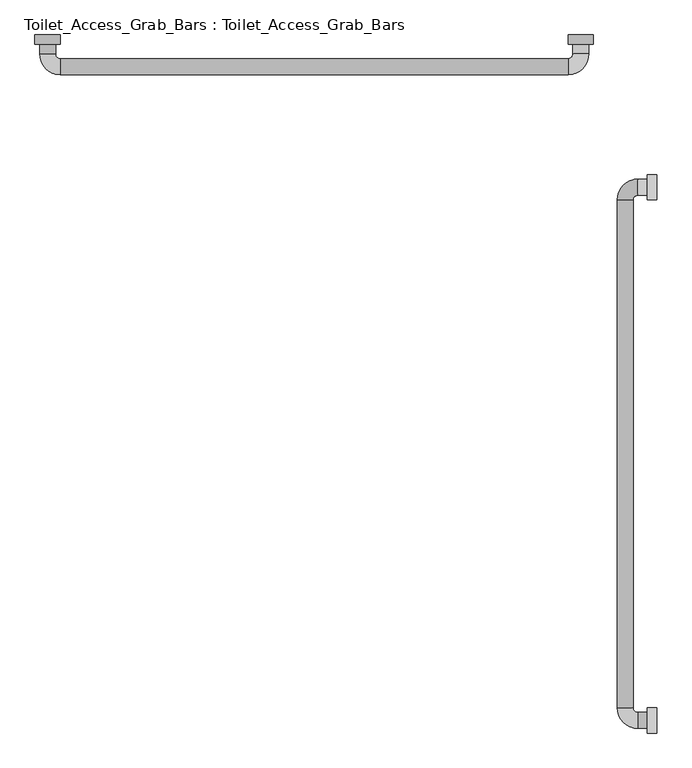
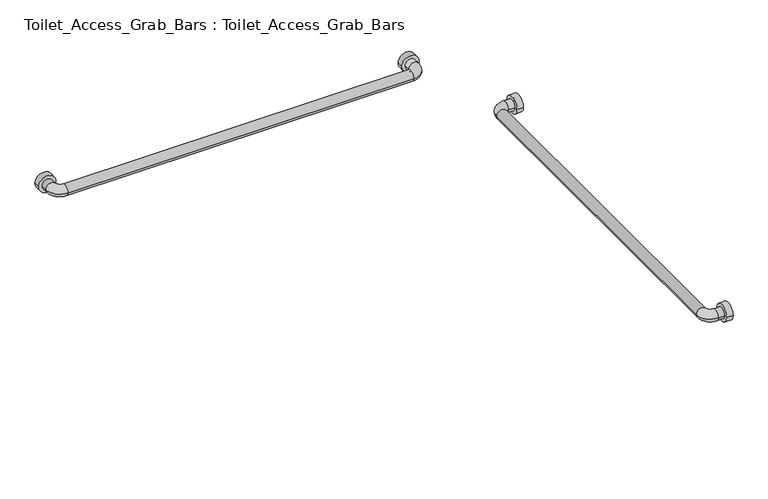
"""IFC4 building model written with IfcOpenShell, lengths in millimetres: proxy geometry, Toilet_Access_Grab_Bars : Toilet_Access_Grab_Bars."""

import ifcopenshell
import ifcopenshell.guid

model = None  # the IFC model being written
_history = None  # IfcOwnerHistory: only IFC2X3 demands one
_inside = {}  # id of a spatial element -> (the spatial element, [elements in it])
_under = {}  # id of a project, library or spatial element -> (it, [spatial elements below it])
_declared = {}  # id of a project -> (the project, [libraries it declares])
_typed = {}  # id of a type object -> (the type object, [elements of that type])
_made_of = {}  # id of a material, layer set ... -> (it, [elements and type objects made of it])


def new_model(schema):
    """Start an empty IFC model of exactly this schema.

    Asked for "IFC4X3", IfcOpenShell would pick the latest addendum, in which some entities
    have other attributes; the version numbers below select the first issue.
    IFC2X3 requires an IfcOwnerHistory on every rooted entity: one is made here for all.
    """
    global model, _history
    if schema == "IFC4X3":
        model = ifcopenshell.file(schema_version=(4, 3, 0, 0))
    else:
        model = ifcopenshell.file(schema=schema)
    _inside.clear()
    _under.clear()
    _declared.clear()
    _typed.clear()
    _made_of.clear()
    _history = None
    if model.schema == "IFC2X3":
        org = make("IfcOrganization", Name="unknown")
        user = make(
            "IfcPersonAndOrganization",
            ThePerson=make("IfcPerson", FamilyName="unknown"),
            TheOrganization=org,
        )
        app = make(
            "IfcApplication",
            ApplicationDeveloper=org,
            Version="unknown",
            ApplicationFullName="unknown",
            ApplicationIdentifier="unknown",
        )
        _history = make(
            "IfcOwnerHistory",
            OwningUser=user,
            OwningApplication=app,
            ChangeAction="ADDED",
            CreationDate=0,
        )
    return model


def make(cls, **values):
    """One entity of the class cls with the attributes given. An attribute that is None is left unset."""
    return model.create_entity(
        cls, **{name: value for name, value in values.items() if value is not None}
    )


def rooted(cls, **values):
    """An entity with a GlobalId (a new one), such as an element, a storey or a relation."""
    return make(cls, GlobalId=ifcopenshell.guid.new(), OwnerHistory=_history, **values)


def si_unit(unit_type, name, prefix=None):
    """IfcSIUnit, for example si_unit("LENGTHUNIT", "METRE", prefix="MILLI")."""
    return make("IfcSIUnit", UnitType=unit_type, Prefix=prefix, Name=name)


def assignment(units):
    """IfcUnitAssignment: the units of a project."""
    return None if units is None else make("IfcUnitAssignment", Units=units)


def point(xyz):
    """IfcCartesianPoint."""
    return None if xyz is None else make("IfcCartesianPoint", Coordinates=xyz)


def direction(xyz):
    """IfcDirection."""
    return None if xyz is None else make("IfcDirection", DirectionRatios=xyz)


def frame(location, z_axis=None, x_axis=None):
    """IfcAxis2Placement3D, a coordinate frame: its origin and axes. An axis left out is left unset."""
    return make(
        "IfcAxis2Placement3D",
        Location=point(location),
        Axis=direction(z_axis),
        RefDirection=direction(x_axis),
    )


def frame_2d(location, x_axis=None):
    """IfcAxis2Placement2D, a coordinate frame in the plane: its origin and x axis."""
    return make(
        "IfcAxis2Placement2D", Location=point(location), RefDirection=direction(x_axis)
    )


def origin():
    """The frame at (0, 0, 0) with its axes left unset."""
    return frame((0.0, 0.0, 0.0))


def place(relative_to, where):
    """IfcLocalPlacement: puts the frame where relative to a parent placement (None: the world)."""
    return make(
        "IfcLocalPlacement", PlacementRelTo=relative_to, RelativePlacement=where
    )


def context(
    kind, dimensions, precision=None, world=None, true_north=None, identifier=None
):
    """IfcGeometricRepresentationContext, for example the 3D "Model" context."""
    return make(
        "IfcGeometricRepresentationContext",
        ContextIdentifier=identifier,
        ContextType=kind,
        CoordinateSpaceDimension=dimensions,
        Precision=precision,
        WorldCoordinateSystem=world,
        TrueNorth=true_north,
    )


def project(units=None, contexts=None):
    """IfcProject with its units and contexts."""
    return rooted(
        "IfcProject",
        Name="project",
        RepresentationContexts=contexts,
        UnitsInContext=assignment(units),
    )


def spatial(cls, under=None, at=None, **own):
    """A site, building, storey or space (cls), placed at a placement, below another one or the project."""
    s = rooted(cls, ObjectPlacement=at, **own)
    if under is not None:
        _under.setdefault(under.id(), (under, []))[1].append(s)
    return s


def circle_curve(where, radius):
    """IfcCircle in the frame where."""
    return make("IfcCircle", Position=where, Radius=radius)


def ellipse_curve(where, semi_axis1, semi_axis2):
    """IfcEllipse in the frame where."""
    return make(
        "IfcEllipse", Position=where, SemiAxis1=semi_axis1, SemiAxis2=semi_axis2
    )


def trimmed(basis, trim1, trim2, sense, master):
    """IfcTrimmedCurve: the piece of a basis curve between two trims."""
    return make(
        "IfcTrimmedCurve",
        BasisCurve=basis,
        Trim1=trim1,
        Trim2=trim2,
        SenseAgreement=sense,
        MasterRepresentation=master,
    )


def segment(curve, same_sense, transition):
    """IfcCompositeCurveSegment."""
    return make(
        "IfcCompositeCurveSegment",
        Transition=transition,
        SameSense=same_sense,
        ParentCurve=curve,
    )


def composite_curve(segments, self_intersect=None):
    """IfcCompositeCurve: segments joined end to end."""
    return make("IfcCompositeCurve", Segments=segments, SelfIntersect=self_intersect)


def outline(outer, holes=None, kind="AREA"):
    """IfcArbitraryClosedProfileDef: a profile drawn as a closed curve; with holes, ...WithVoids."""
    if holes is None:
        return make("IfcArbitraryClosedProfileDef", ProfileType=kind, OuterCurve=outer)
    return make(
        "IfcArbitraryProfileDefWithVoids",
        ProfileType=kind,
        OuterCurve=outer,
        InnerCurves=holes,
    )


def extrude(swept, where, along, depth):
    """IfcExtrudedAreaSolid: the profile swept, set in the frame where, extruded along a direction by depth."""
    return make(
        "IfcExtrudedAreaSolid",
        SweptArea=swept,
        Position=where,
        ExtrudedDirection=direction(along),
        Depth=depth,
    )


def shape(context_of_items, identifier, shape_type, items):
    """IfcShapeRepresentation: the items that make up one representation, for example the "Body"."""
    return make(
        "IfcShapeRepresentation",
        ContextOfItems=context_of_items,
        RepresentationIdentifier=identifier,
        RepresentationType=shape_type,
        Items=items,
    )


def source(mapping_origin, context_of_items, identifier, shape_type, items):
    """IfcRepresentationMap: a shape defined once, which mapped items show again and again."""
    return make(
        "IfcRepresentationMap",
        MappingOrigin=mapping_origin,
        MappedRepresentation=shape(context_of_items, identifier, shape_type, items),
    )


def transform(
    local_origin,
    x_axis=None,
    y_axis=None,
    z_axis=None,
    scale=None,
    scale2=None,
    scale3=None,
    uniform=True,
):
    """IfcCartesianTransformationOperator3D, or its non-uniform kind. x_axis, y_axis, z_axis: its Axis1, 2, 3."""
    if uniform:
        return make(
            "IfcCartesianTransformationOperator3D",
            Axis1=direction(x_axis),
            Axis2=direction(y_axis),
            LocalOrigin=point(local_origin),
            Scale=scale,
            Axis3=direction(z_axis),
        )
    return make(
        "IfcCartesianTransformationOperator3DnonUniform",
        Axis1=direction(x_axis),
        Axis2=direction(y_axis),
        LocalOrigin=point(local_origin),
        Scale=scale,
        Axis3=direction(z_axis),
        Scale2=scale2,
        Scale3=scale3,
    )


def mapped(mapping_source, mapping_target):
    """IfcMappedItem: shows the shape of a source again, moved by a transform."""
    return make(
        "IfcMappedItem", MappingSource=mapping_source, MappingTarget=mapping_target
    )


def made_of(thing, what):
    """Note that an element or type object is made of a material, layer set ...; save() writes the relation."""
    if what is not None:
        _made_of.setdefault(what.id(), (what, []))[1].append(thing)
    return thing


def element(
    cls,
    number,
    at=None,
    inside=None,
    cuts=None,
    type_object=None,
    material=None,
    context=None,
    identifier="Body",
    shape_type=None,
    held_by="IfcProductDefinitionShape",
    body=None,
    shapes=None,
    **own,
):
    """One element of the class cls, such as IfcWall. Its Tag is "e" and its number.

    at: its placement. inside: the storey or other place that contains it. cuts: it is an
    opening in that element (IfcRelVoidsElement). A single representation is given by context,
    identifier, shape_type and body (its items); several are given by shapes. held_by: the class
    of the entity that holds the representations. save() writes the other relations.
    """
    e = rooted(cls, Tag="e%d" % number, ObjectPlacement=at, **own)
    if body is not None:
        shapes = [shape(context, identifier, shape_type, body)]
    if shapes is not None:
        e.Representation = make(held_by, Representations=shapes)
    if inside is not None:
        _inside.setdefault(inside.id(), (inside, []))[1].append(e)
    if cuts is not None:
        rooted(
            "IfcRelVoidsElement", RelatingBuildingElement=cuts, RelatedOpeningElement=e
        )
    if type_object is not None:
        _typed.setdefault(type_object.id(), (type_object, []))[1].append(e)
    return made_of(e, material)


def aggregate(whole, parts):
    """IfcRelAggregates: a whole, such as a stair, and the parts it consists of."""
    return rooted("IfcRelAggregates", RelatingObject=whole, RelatedObjects=parts)


def save(model, path):
    """Write the relations noted so far, then the file.

    IfcRelAggregates (storeys below a building ...), IfcRelContainedInSpatialStructure (elements
    in a storey), IfcRelDefinesByType, IfcRelAssociatesMaterial and IfcRelDeclares: one each for
    every whole, place, type object, material and project.
    """
    for whole, parts in _under.values():
        aggregate(whole, parts)
    for where, things in _inside.values():
        rooted(
            "IfcRelContainedInSpatialStructure",
            RelatedElements=things,
            RelatingStructure=where,
        )
    for kind, things in _typed.values():
        rooted("IfcRelDefinesByType", RelatedObjects=things, RelatingType=kind)
    for what, things in _made_of.values():
        rooted("IfcRelAssociatesMaterial", RelatedObjects=things, RelatingMaterial=what)
    for by, libraries in _declared.values():
        rooted("IfcRelDeclares", RelatingContext=by, RelatedDefinitions=libraries)
    model.write(path)


def plane_surface(at):
    """IfcPlane: the flat surface through the origin of the frame at, square to its z axis."""
    return make("IfcPlane", Position=at)


def cylinder_surface(at, radius):
    """IfcCylindricalSurface: all points at the distance radius from the z axis of the frame at."""
    return make("IfcCylindricalSurface", Position=at, Radius=radius)


def revolved_surface(curve, axis_point, axis_direction):
    """IfcSurfaceOfRevolution: the curve turned about the line through axis_point along axis_direction."""
    return make(
        "IfcSurfaceOfRevolution",
        SweptCurve=make("IfcArbitraryOpenProfileDef", ProfileType="CURVE", Curve=curve),
        AxisPosition=make("IfcAxis1Placement", Location=point(axis_point), Axis=direction(axis_direction)),
    )


def advanced_brep(points, edges, surfaces, faces):
    """IfcAdvancedBrep: a solid bounded by faces that lie on surfaces and meet in shared edges.

    An edge is (start, end): straight between two places in points (the first is 0);
    or (start, end, curve); or (start, end, curve, False) where it runs against its curve.
    A face is (place in surfaces, loops), or (place, loops, False) where it looks against
    its surface's normal. A loop lists edges by number (the first is 1), with a minus sign
    where the edge is run from its end to its start. The first loop is the outer one.
    """
    corners = [point(p) for p in points]
    vertices = [make("IfcVertexPoint", VertexGeometry=c) for c in corners]
    made = []
    for start, end, *more in edges:
        made.append(
            make(
                "IfcEdgeCurve",
                EdgeStart=vertices[start],
                EdgeEnd=vertices[end],
                EdgeGeometry=more[0] if more else make("IfcPolyline", Points=[corners[start], corners[end]]),
                SameSense=more[1] if len(more) > 1 else True,
            )
        )
    hull = []
    for where, loops, *sense in faces:
        bounds = []
        for j, loop in enumerate(loops):
            ring = [make("IfcOrientedEdge", EdgeElement=made[abs(k) - 1], Orientation=k > 0) for k in loop]
            bounds.append(
                make(
                    "IfcFaceOuterBound" if j == 0 else "IfcFaceBound",
                    Bound=make("IfcEdgeLoop", EdgeList=ring),
                    Orientation=True,
                )
            )
        hull.append(make("IfcAdvancedFace", Bounds=bounds, FaceSurface=surfaces[where], SameSense=sense[0] if sense else True))
    return make("IfcAdvancedBrep", Outer=make("IfcClosedShell", CfsFaces=hull))


def toilet_access_grab_bars_toilet_access_grab_bars_ef23dea8(model_context):
    return source(origin(), model_context, "Body", "SolidModel", [
        extrude(outline(composite_curve([segment(trimmed(circle_curve(frame_2d((-304.8, 838.2)), 25.4), [point((-279.4, 838.2))], [point((-330.2, 838.2))], False, "CARTESIAN"), True, "CONTINUOUS"), segment(trimmed(circle_curve(frame_2d((-304.8, 838.2)), 25.4), [point((-330.2, 838.2))], [point((-279.4, 838.2))], False, "CARTESIAN"), True, "CONTINUOUS")], self_intersect=False)), frame((-19.05, 0.0, 0.0), z_axis=(1.0, 0.0, 0.0), x_axis=(0.0, 1.0, 0.0)), (0.0, 0.0, 1.0), 19.05),
        extrude(outline(composite_curve([segment(trimmed(circle_curve(frame_2d((-1371.6, 838.2)), 25.4), [point((-1346.2, 838.2))], [point((-1397.0, 838.2))], False, "CARTESIAN"), True, "CONTINUOUS"), segment(trimmed(circle_curve(frame_2d((-1371.6, 838.2)), 25.4), [point((-1397.0, 838.2))], [point((-1346.2, 838.2))], False, "CARTESIAN"), True, "CONTINUOUS")], self_intersect=False)), frame((-19.05, 0.0, 0.0), z_axis=(1.0, 0.0, 0.0), x_axis=(0.0, 1.0, 0.0)), (0.0, 0.0, 1.0), 19.05),
        extrude(outline(composite_curve([segment(trimmed(circle_curve(frame_2d((838.2, -152.4)), 25.4), [point((838.2, -177.8))], [point((838.2, -127.0))], False, "CARTESIAN"), True, "CONTINUOUS"), segment(trimmed(circle_curve(frame_2d((838.2, -152.4)), 25.4), [point((838.2, -127.0))], [point((838.2, -177.8))], False, "CARTESIAN"), True, "CONTINUOUS")], self_intersect=False)), frame((0.0, -19.05, 0.0), z_axis=(0.0, 1.0, 0.0), x_axis=(0.0, 0.0, 1.0)), (0.0, 0.0, 1.0), 19.05),
        extrude(outline(composite_curve([segment(trimmed(circle_curve(frame_2d((838.2, -1219.2)), 25.4), [point((838.2, -1244.6))], [point((838.2, -1193.8))], False, "CARTESIAN"), True, "CONTINUOUS"), segment(trimmed(circle_curve(frame_2d((838.2, -1219.2)), 25.4), [point((838.2, -1193.8))], [point((838.2, -1244.6))], False, "CARTESIAN"), True, "CONTINUOUS")], self_intersect=False)), frame((0.0, -19.05, 0.0), z_axis=(0.0, 1.0, 0.0), x_axis=(0.0, 0.0, 1.0)), (0.0, 0.0, 1.0), 19.05),
        advanced_brep(
        [(-19.05, -320.675, 838.2), (-19.05, -288.925, 838.2), (-38.1, -288.925, 838.2), (-38.1, -320.675, 838.2), (-79.375, -330.2, 838.2), (-47.625, -330.2, 838.2), (-79.375, -1346.2, 838.2), (-47.625, -1346.2, 838.2), (-38.1, -1387.475, 838.2), (-38.1, -1355.725, 838.2), (-19.05, -1355.725, 838.2), (-19.05, -1387.475, 838.2)],
        [
            (0, 1, circle_curve(frame((-19.05, -304.8, 838.2), z_axis=(1.0, 0.0, 0.0), x_axis=(0.0, 1.0, 0.0)), 15.875)),
            (1, 0, circle_curve(frame((-19.05, -304.8, 838.2), z_axis=(1.0, 0.0, 0.0), x_axis=(0.0, 1.0, 0.0)), 15.875)),
            (1, 2),
            (2, 3, circle_curve(frame((-38.1, -304.8, 838.2), z_axis=(1.0, 0.0, 0.0), x_axis=(0.0, 1.0, 0.0)), 15.875)),
            (3, 0),
            (3, 2, circle_curve(frame((-38.1, -304.8, 838.2), z_axis=(1.0, 0.0, 0.0), x_axis=(0.0, 1.0, 0.0)), 15.875)),
            (4, 5, circle_curve(frame((-63.5, -330.2, 838.2), z_axis=(0.0, 1.0, 0.0), x_axis=(-1.0, 0.0, 0.0)), 15.875)),
            (5, 3, circle_curve(frame((-38.1, -330.2, 838.2), z_axis=(0.0, 0.0, -1.0), x_axis=(0.0, 1.0, 0.0)), 9.525)),
            (2, 4, circle_curve(frame((-38.1, -330.2, 838.2), z_axis=(0.0, 0.0, 1.0), x_axis=(0.0, 1.0, 0.0)), 41.275)),
            (5, 4, circle_curve(frame((-63.5, -330.2, 838.2), z_axis=(0.0, 1.0, 0.0), x_axis=(-1.0, 0.0, 0.0)), 15.875)),
            (4, 6),
            (6, 7, circle_curve(frame((-63.5, -1346.2, 838.2), z_axis=(0.0, 1.0, 0.0), x_axis=(-1.0, 0.0, 0.0)), 15.875)),
            (7, 5),
            (7, 6, circle_curve(frame((-63.5, -1346.2, 838.2), z_axis=(0.0, 1.0, 0.0), x_axis=(-1.0, 0.0, 0.0)), 15.875)),
            (8, 9, circle_curve(frame((-38.1, -1371.6, 838.2), z_axis=(-1.0, 0.0, 0.0), x_axis=(0.0, -1.0, 0.0)), 15.875)),
            (9, 7, circle_curve(frame((-38.1, -1346.2, 838.2), z_axis=(0.0, 0.0, -1.0), x_axis=(-1.0, 0.0, 0.0)), 9.525)),
            (6, 8, circle_curve(frame((-38.1, -1346.2, 838.2), z_axis=(0.0, 0.0, 1.0), x_axis=(-1.0, 0.0, 0.0)), 41.275)),
            (9, 8, circle_curve(frame((-38.1, -1371.6, 838.2), z_axis=(-1.0, 0.0, 0.0), x_axis=(0.0, -1.0, 0.0)), 15.875)),
            (10, 11, circle_curve(frame((-19.05, -1371.6, 838.2), z_axis=(1.0, 0.0, 0.0), x_axis=(0.0, -1.0, 0.0)), 15.875)),
            (11, 10, circle_curve(frame((-19.05, -1371.6, 838.2), z_axis=(1.0, 0.0, 0.0), x_axis=(0.0, -1.0, 0.0)), 15.875)),
            (8, 11),
            (10, 9),
        ],
        [
            plane_surface(frame((-19.05, -304.8, -854.075), z_axis=(1.0, 0.0, 0.0), x_axis=(0.0, 1.0, 0.0))),
            cylinder_surface(frame((-19.05, -304.8, 838.2), z_axis=(1.0, 0.0, 0.0), x_axis=(0.0, 1.0, 0.0)), 15.875),
            revolved_surface(trimmed(ellipse_curve(frame((-38.1, -304.8, 838.2), z_axis=(-1.0, 0.0, 0.0), x_axis=(0.0, 1.0, 0.0)), 15.875, 15.875), [point((-38.1, -320.675, 838.2))], [point((-38.1, -288.925, 838.2))], True, "CARTESIAN"), (-38.1, -330.2, 0.0), (0.0, 0.0, -1.0)),
            revolved_surface(trimmed(ellipse_curve(frame((-38.1, -304.8, 838.2), z_axis=(-1.0, 0.0, 0.0), x_axis=(0.0, 1.0, 0.0)), 15.875, 15.875), [point((-38.1, -288.925, 838.2))], [point((-38.1, -320.675, 838.2))], True, "CARTESIAN"), (-38.1, -330.2, 0.0), (0.0, 0.0, -1.0)),
            cylinder_surface(frame((-63.5, -330.2, 838.2), z_axis=(0.0, 1.0, 0.0), x_axis=(-1.0, 0.0, 0.0)), 15.875),
            revolved_surface(trimmed(ellipse_curve(frame((-63.5, -1346.2, 838.2), z_axis=(0.0, -1.0, 0.0), x_axis=(-1.0, 0.0, 0.0)), 15.875, 15.875), [point((-47.625, -1346.2, 838.2))], [point((-79.375, -1346.2, 838.2))], True, "CARTESIAN"), (-38.1, -1346.2, 0.0), (0.0, 0.0, -1.0)),
            revolved_surface(trimmed(ellipse_curve(frame((-63.5, -1346.2, 838.2), z_axis=(0.0, -1.0, 0.0), x_axis=(-1.0, 0.0, 0.0)), 15.875, 15.875), [point((-79.375, -1346.2, 838.2))], [point((-47.625, -1346.2, 838.2))], True, "CARTESIAN"), (-38.1, -1346.2, 0.0), (0.0, 0.0, -1.0)),
            plane_surface(frame((-19.05, -1371.6, -854.075), z_axis=(1.0, 0.0, 0.0), x_axis=(0.0, -1.0, 0.0))),
            cylinder_surface(frame((-38.1, -1371.6, 838.2), z_axis=(-1.0, 0.0, 0.0), x_axis=(0.0, -1.0, 0.0)), 15.875),
        ],
        [
            (0, [[1, 2]]),
            (1, [[3, 4, 5, -2]]),
            (1, [[-5, 6, -3, -1]]),
            (2, [[7, 8, -4, 9]]),
            (3, [[10, -9, -6, -8]]),
            (4, [[11, 12, 13, -7]]),
            (4, [[-13, 14, -11, -10]]),
            (5, [[15, 16, -12, 17]]),
            (6, [[18, -17, -14, -16]]),
            (7, [[19, 20]]),
            (8, [[21, -19, 22, -15]]),
            (8, [[-22, -20, -21, -18]]),
        ],
    ),
        advanced_brep(
        [(-1203.325, -19.05, 838.2), (-1235.075, -19.05, 838.2), (-1235.075, -38.1, 838.2), (-1203.325, -38.1, 838.2), (-1193.8, -79.375, 838.2), (-1193.8, -47.625, 838.2), (-177.8, -79.375, 838.2), (-177.8, -47.625, 838.2), (-136.525, -38.1, 838.2), (-168.275, -38.1, 838.2), (-168.275, -19.05, 838.2), (-136.525, -19.05, 838.2)],
        [
            (0, 1, circle_curve(frame((-1219.2, -19.05, 838.2), z_axis=(0.0, 1.0, 0.0), x_axis=(-1.0, 0.0, 0.0)), 15.875)),
            (1, 0, circle_curve(frame((-1219.2, -19.05, 838.2), z_axis=(0.0, 1.0, 0.0), x_axis=(-1.0, 0.0, 0.0)), 15.875)),
            (1, 2),
            (2, 3, circle_curve(frame((-1219.2, -38.1, 838.2), z_axis=(0.0, 1.0, 0.0), x_axis=(-1.0, 0.0, 0.0)), 15.875)),
            (3, 0),
            (3, 2, circle_curve(frame((-1219.2, -38.1, 838.2), z_axis=(0.0, 1.0, 0.0), x_axis=(-1.0, 0.0, 0.0)), 15.875)),
            (4, 5, circle_curve(frame((-1193.8, -63.5, 838.2), z_axis=(-1.0, 0.0, 0.0), x_axis=(0.0, -1.0, 0.0)), 15.875)),
            (5, 3, circle_curve(frame((-1193.8, -38.1, 838.2), z_axis=(0.0, 0.0, -1.0), x_axis=(-1.0, 0.0, 0.0)), 9.525)),
            (2, 4, circle_curve(frame((-1193.8, -38.1, 838.2), z_axis=(0.0, 0.0, 1.0), x_axis=(-1.0, 0.0, 0.0)), 41.275)),
            (5, 4, circle_curve(frame((-1193.8, -63.5, 838.2), z_axis=(-1.0, 0.0, 0.0), x_axis=(0.0, -1.0, 0.0)), 15.875)),
            (4, 6),
            (6, 7, circle_curve(frame((-177.8, -63.5, 838.2), z_axis=(-1.0, 0.0, 0.0), x_axis=(0.0, -1.0, 0.0)), 15.875)),
            (7, 5),
            (7, 6, circle_curve(frame((-177.8, -63.5, 838.2), z_axis=(-1.0, 0.0, 0.0), x_axis=(0.0, -1.0, 0.0)), 15.875)),
            (8, 9, circle_curve(frame((-152.4, -38.1, 838.2), z_axis=(0.0, -1.0, 0.0), x_axis=(1.0, 0.0, 0.0)), 15.875)),
            (9, 7, circle_curve(frame((-177.8, -38.1, 838.2), z_axis=(0.0, 0.0, -1.0), x_axis=(0.0, -1.0, 0.0)), 9.525)),
            (6, 8, circle_curve(frame((-177.8, -38.1, 838.2), z_axis=(0.0, 0.0, 1.0), x_axis=(0.0, -1.0, 0.0)), 41.275)),
            (9, 8, circle_curve(frame((-152.4, -38.1, 838.2), z_axis=(0.0, -1.0, 0.0), x_axis=(1.0, 0.0, 0.0)), 15.875)),
            (10, 11, circle_curve(frame((-152.4, -19.05, 838.2), z_axis=(0.0, 1.0, 0.0), x_axis=(1.0, 0.0, 0.0)), 15.875)),
            (11, 10, circle_curve(frame((-152.4, -19.05, 838.2), z_axis=(0.0, 1.0, 0.0), x_axis=(1.0, 0.0, 0.0)), 15.875)),
            (8, 11),
            (10, 9),
        ],
        [
            plane_surface(frame((-2073.275, -19.05, 0.0), z_axis=(0.0, 1.0, 0.0), x_axis=(0.0, 0.0, 1.0))),
            cylinder_surface(frame((-1219.2, -19.05, 838.2), z_axis=(0.0, 1.0, 0.0), x_axis=(-1.0, 0.0, 0.0)), 15.875),
            revolved_surface(trimmed(ellipse_curve(frame((-1219.2, -38.1, 838.2), z_axis=(0.0, -1.0, 0.0), x_axis=(-1.0, 0.0, 0.0)), 15.875, 15.875), [point((-1203.325, -38.1, 838.2))], [point((-1235.075, -38.1, 838.2))], True, "CARTESIAN"), (-1193.8, -38.1, 0.0), (0.0, 0.0, -1.0)),
            revolved_surface(trimmed(ellipse_curve(frame((-1219.2, -38.1, 838.2), z_axis=(0.0, -1.0, 0.0), x_axis=(-1.0, 0.0, 0.0)), 15.875, 15.875), [point((-1235.075, -38.1, 838.2))], [point((-1203.325, -38.1, 838.2))], True, "CARTESIAN"), (-1193.8, -38.1, 0.0), (0.0, 0.0, -1.0)),
            cylinder_surface(frame((-1193.8, -63.5, 838.2), z_axis=(-1.0, 0.0, 0.0), x_axis=(0.0, -1.0, 0.0)), 15.875),
            revolved_surface(trimmed(ellipse_curve(frame((-177.8, -63.5, 838.2), z_axis=(1.0, 0.0, 0.0), x_axis=(0.0, -1.0, 0.0)), 15.875, 15.875), [point((-177.8, -47.625, 838.2))], [point((-177.8, -79.375, 838.2))], True, "CARTESIAN"), (-177.8, -38.1, 0.0), (0.0, 0.0, -1.0)),
            revolved_surface(trimmed(ellipse_curve(frame((-177.8, -63.5, 838.2), z_axis=(1.0, 0.0, 0.0), x_axis=(0.0, -1.0, 0.0)), 15.875, 15.875), [point((-177.8, -79.375, 838.2))], [point((-177.8, -47.625, 838.2))], True, "CARTESIAN"), (-177.8, -38.1, 0.0), (0.0, 0.0, -1.0)),
            plane_surface(frame((-1006.475, -19.05, 0.0), z_axis=(0.0, 1.0, 0.0), x_axis=(0.0, 0.0, -1.0))),
            cylinder_surface(frame((-152.4, -38.1, 838.2), z_axis=(0.0, -1.0, 0.0), x_axis=(1.0, 0.0, 0.0)), 15.875),
        ],
        [
            (0, [[1, 2]]),
            (1, [[3, 4, 5, -2]]),
            (1, [[-5, 6, -3, -1]]),
            (2, [[7, 8, -4, 9]]),
            (3, [[10, -9, -6, -8]]),
            (4, [[11, 12, 13, -7]]),
            (4, [[-13, 14, -11, -10]]),
            (5, [[15, 16, -12, 17]]),
            (6, [[18, -17, -14, -16]]),
            (7, [[19, 20]]),
            (8, [[21, -19, 22, -15]]),
            (8, [[-22, -20, -21, -18]]),
        ],
    ),
    ])


if __name__ == "__main__":
    model = new_model("IFC4")
    model_context = context("Model", 3, world=origin())
    ifc_project = project(units=[si_unit("LENGTHUNIT", "METRE", prefix="MILLI")], contexts=[model_context])
    site = spatial("IfcSite", under=ifc_project)
    building = spatial("IfcBuilding", under=site)
    placement = place(None, origin())
    toilet_access_grab_bars_toilet_access_grab_bars_shape = toilet_access_grab_bars_toilet_access_grab_bars_ef23dea8(model_context)
    element("IfcBuildingElementProxy", 1, Name="Toilet_Access_Grab_Bars : Toilet_Access_Grab_Bars", ObjectType="Toilet_Access_Grab_Bars : Toilet_Access_Grab_Bars", at=placement, inside=building, context=model_context, shape_type="MappedRepresentation", body=[
        mapped(toilet_access_grab_bars_toilet_access_grab_bars_shape, transform((0.0, 0.0, 0.0), x_axis=(1.0, 0.0, 0.0), y_axis=(0.0, 1.0, 0.0), z_axis=(0.0, 0.0, 1.0))),
    ])
    save(model, "model.ifc")

# Revit data of these elements
# Type "Toilet_Access_Grab_Bars : Toilet_Access_Grab_Bars"
#   Back Bar Length = 3' - 6"
#   Mounting Height = 2' - 9"
#   Side Bar Length = 3' - 6"
#   Default Elevation = 0
#   Assembly Code = ""
# Element 1 (IfcBuildingElementProxy, "Toilet_Access_Grab_Bars : Toilet_Access_Grab_Bars")
#   Materials on its faces: "Metal - Aluminum, Brushed"
# Materials
#   "Metal - Aluminum, Brushed": class "Unassigned", colour RGB 247 247 247, transparency 0
